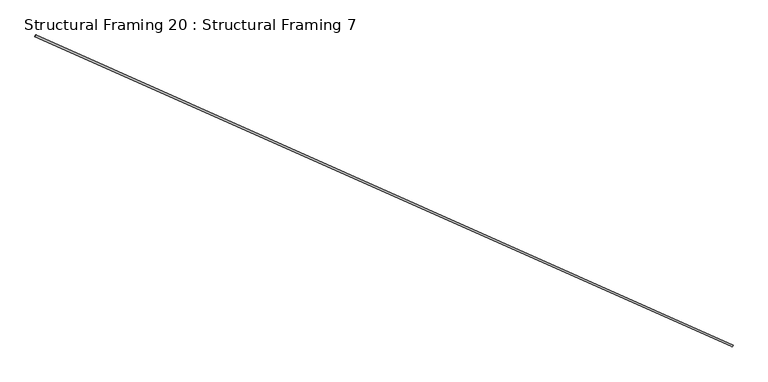
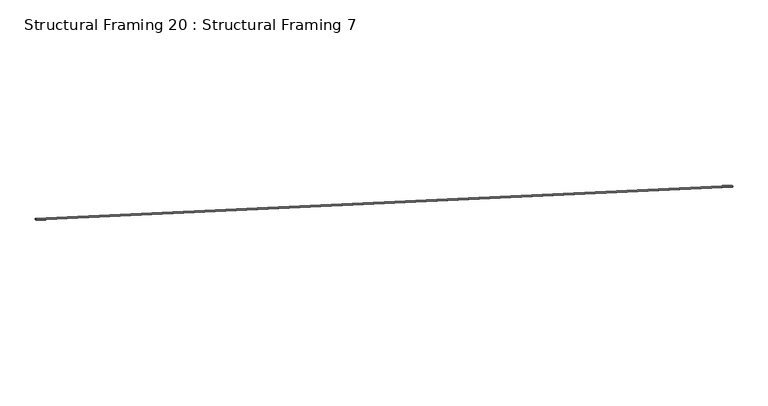
"""IFC4 building model written with IfcOpenShell, lengths in millimetres: beam geometry, Structural Framing 20 : Structural Framing 7."""

from ifc_helpers import new_model, si_unit, point, frame, origin, origin_2d, place, context, project, spatial, circle_curve, trimmed, segment, composite_curve, outline, extrude, source, transform, mapped, element, save


def structural_framing_20_structural_framing_7_b793b059(model_context):
    return source(origin(), model_context, "Body", "SweptSolid", [
        extrude(outline(composite_curve([segment(trimmed(circle_curve(origin_2d(), 6.35), [point((-1e-07, 6.3500001))], [point((0.0, -6.35))], False, "CARTESIAN"), True, "CONTINUOUS"), segment(trimmed(circle_curve(origin_2d(), 6.35), [point((0.0, -6.35))], [point((-1e-07, 6.3500001))], False, "CARTESIAN"), True, "CONTINUOUS")], self_intersect=False)), frame((30023.5870052, 270.9973838, 2860.5759358), z_axis=(-0.9135454576426018, 0.40642988240442374, 0.015793907347322014), x_axis=(0.0, 0.03883079534680305, -0.9992458002577418)), (0.0, 0.0, 1.0), 5505.1447719),
    ])


if __name__ == "__main__":
    model = new_model("IFC4")
    model_context = context("Model", 3, world=origin())
    ifc_project = project(units=[si_unit("LENGTHUNIT", "METRE", prefix="MILLI")], contexts=[model_context])
    site = spatial("IfcSite", under=ifc_project)
    building = spatial("IfcBuilding", under=site)
    placement = place(None, origin())
    structural_framing_20_structural_framing_7_shape = structural_framing_20_structural_framing_7_b793b059(model_context)
    element("IfcBeam", 1, ObjectType="Structural Framing 20 : Structural Framing 7", at=placement, inside=building, context=model_context, shape_type="MappedRepresentation", body=[
        mapped(structural_framing_20_structural_framing_7_shape, transform((0.0, 0.0, 0.0), x_axis=(1.0, 0.0, 0.0), y_axis=(0.0, 1.0, 0.0), z_axis=(0.0, 0.0, 1.0))),
    ])
    save(model, "model.ifc")

# Revit data of these elements
# Type "Structural Framing 20 : Structural Framing 7"
#   Structural Material [instance default] = EXISTING LATERAL BRACING (1/4" CABLE)
# Element 1 (IfcBeam, "Structural Framing 20 : Structural Framing 7")
#   Materials on its faces: "EXISTING LATERAL BRACING (1/4\" CABLE)"
# Materials
#   "EXISTING LATERAL BRACING (1/4\" CABLE)": class "Generic", colour RGB 120 120 120, transparency 0, Cost = 0
